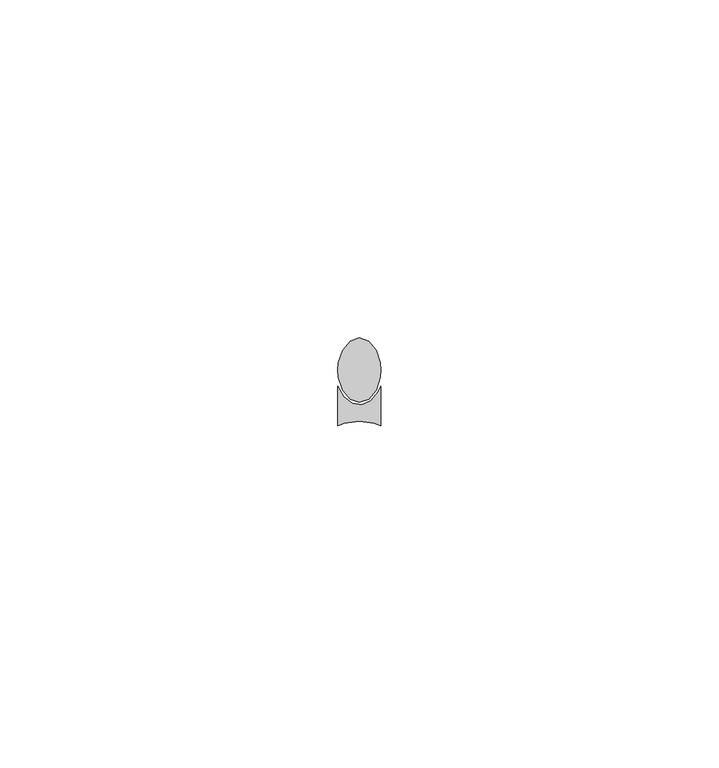
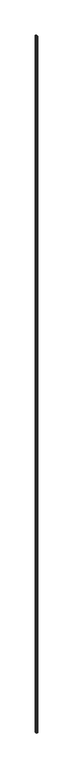
"""IFC4 building model written with IfcOpenShell, lengths in millimetres: proxy geometry, Generic Models 11:Generic Models 1:306267:Generic Models 1:306267 : Generic Models 11:Generic Models 1:306267:300405:Generic Models 1:306267:Generic Models 1:306267 : Generic Models 11:Generic Models 1:306267:300405 : Generic Models 11:Generic Models 1:306267:Generic Models 1:306267 : Generic Models 11:Generic Models 1:306267:300405:23 : Generic Models 11:Generic Models 1:306267:Generic Models 1:306267 : Generic Models 11:Generic Models 1:306267:300405:Generic Models 1:306267:Generic Models 1:306267 : Generic Models 11:Generic Models 1:306267:300405 : Generic Models 11:Generic Models 1:306267:Generic Models 1:306267 : Generic Models 11:Generic Models 1:306267:300405:300182."""

from ifc_helpers import new_model, si_unit, frame, origin, place, context, project, spatial, polyline, outline, extrude, source, transform, mapped, element, save


def generic_models_3989d67e(model_context):
    return source(origin(), model_context, "Body", "SweptSolid", [
        extrude(outline(polyline([(594928.7897638, -579082.4586403), (594927.4121829, -579082.9302761), (594926.034602, -579082.4586403), (594924.929868, -579081.1371463), (594924.3167868, -579079.2275321), (594924.2371829, -579078.1677761), (594924.3167868, -579077.1080202), (594924.929868, -579075.1984059), (594926.034602, -579073.8769119), (594927.4121829, -579073.4052761), (594928.7897638, -579073.8769119), (594929.8944979, -579075.1984059), (594930.507579, -579077.1080202), (594930.5871829, -579078.1677761), (594930.507579, -579079.2275321), (594929.8944979, -579081.1371463), (594928.7897638, -579082.4586403)])), frame((0.0, 0.0, 31.75), z_axis=(0.0, 0.0, 1.0), x_axis=(1.0, 0.0, 0.0)), (0.0, 0.0, 1.0), 3663.95),
        extrude(outline(polyline([(594925.2029461, -579086.0220872), (594924.2371829, -579086.3994958), (594924.2371829, -579080.5314037), (594925.1199717, -579082.1246204), (594926.3613558, -579083.0988254), (594927.7671321, -579083.3016133), (594929.1173799, -579082.7012598), (594930.2008653, -579081.3916847), (594930.5871829, -579080.5314037), (594930.5871829, -579086.3994958), (594929.6214197, -579086.0220872), (594927.4121829, -579085.7084011), (594925.2029461, -579086.0220872)])), frame((0.0, 0.0, 31.75), z_axis=(0.0, 0.0, 1.0), x_axis=(1.0, 0.0, 0.0)), (0.0, 0.0, 1.0), 3663.95),
    ])


if __name__ == "__main__":
    model = new_model("IFC4")
    model_context = context("Model", 3, world=origin())
    ifc_project = project(units=[si_unit("LENGTHUNIT", "METRE", prefix="MILLI")], contexts=[model_context])
    site = spatial("IfcSite", under=ifc_project)
    building = spatial("IfcBuilding", under=site)
    placement = place(None, origin())
    generic_models_shape = generic_models_3989d67e(model_context)
    element("IfcBuildingElementProxy", 1, Name="Generic Models 11:Generic Models 1:306267:Generic Models 1:306267 : Generic Models 11:Generic Models 1:306267:300405:Generic Models 1:306267:Generic Models 1:306267 : Generic Models 11:Generic Models 1:306267:300405 : Generic Models 11:Generic Models 1:306267:Generic Models 1:306267 : Generic Models 11:Generic Models 1:306267:300405:23 : Generic Models 11:Generic Models 1:306267:Generic Models 1:306267 : Generic Models 11:Generic Models 1:306267:300405:Generic Models 1:306267:Generic Models 1:306267 : Generic Models 11:Generic Models 1:306267:300405 : Generic Models 11:Generic Models 1:306267:Generic Models 1:306267 : Generic Models 11:Generic Models 1:306267:300405:300182", ObjectType="Generic Models 11:Generic Models 1:306267:Generic Models 1:306267 : Generic Models 11:Generic Models 1:306267:300405:Generic Models 1:306267:Generic Models 1:306267 : Generic Models 11:Generic Models 1:306267:300405 : Generic Models 11:Generic Models 1:306267:Generic Models 1:306267 : Generic Models 11:Generic Models 1:306267:300405:23 : Generic Models 11:Generic Models 1:306267:Generic Models 1:306267 : Generic Models 11:Generic Models 1:306267:300405:Generic Models 1:306267:Generic Models 1:306267 : Generic Models 11:Generic Models 1:306267:300405 : Generic Models 11:Generic Models 1:306267:Generic Models 1:306267 : Generic Models 11:Generic Models 1:306267:300405:300182", at=placement, inside=building, context=model_context, shape_type="MappedRepresentation", body=[
        mapped(generic_models_shape, transform((0.0, 0.0, 0.0), x_axis=(1.0, 0.0, 0.0), y_axis=(0.0, 1.0, 0.0), z_axis=(0.0, 0.0, 1.0))),
    ])
    save(model, "model.ifc")

# Revit data of these elements
# Type "Generic Models 11:Generic Models 1:306267:Generic Models 1:306267 : Generic Models 11:Generic Models 1:306267:300405:Generic Models 1:306267:Generic Models 1:306267 : Generic Models 11:Generic Models 1:306267:300405 : Generic Models 11:Generic Models 1:306267:Generic Models 1:306267 : Generic Models 11:Generic Models 1:306267:300405:23 : Generic Models 11:Generic Models 1:306267:Generic Models 1:306267 : Generic Models 11:Generic Models 1:306267:300405:Generic Models 1:306267:Generic Models 1:306267 : Generic Models 11:Generic Models 1:306267:300405 : Generic Models 11:Generic Models 1:306267:Generic Models 1:306267 : Generic Models 11:Generic Models 1:306267:300405:300182"
#   NameOverride = "Generic Models 11:Generic Models 1:306267:Generic Models 1:306267 : Generic Models 11:Generic Models 1:306267:300405:Generic Models 1:306267:Generic Models 1:306267 : Generic Models 11:Generic Models 1:306267:300405 : Generic Models 11:Generic Models 1:306267:Generic Models 1:306267 : Generic Models 11:Generic Models 1:306267:300405:300182"
#   ObjectTypeOverride = "Generic Models 1:306267:Generic Models 1:306267 : Generic Models 11:Generic Models 1:306267:300405 : Generic Models 11:Generic Models 1:306267:Generic Models 1:306267 : Generic Models 11:Generic Models 1:306267:300405"
#   Reference = "Generic Models 1"
#   Tag = "300182"
# Element 1 (IfcBuildingElementProxy, "Generic Models 11:Generic Models 1:306267:Generic Models 1:306267 : Generic Models 11:Generic Models 1:306267:300405:Generic Models 1:306267:Generic Models 1:306267 : Generic Models 11:Generic Models 1:306267:300405 : Generic Models 11:Generic Models 1:306267:Generic Models 1:306267 : Generic Models 11:Generic Models 1:306267:300405:23 : Generic Models 11:Generic Models 1:306267:Generic Models 1:306267 : Generic Models 11:Generic Models 1:306267:300405:Generic Models 1:306267:Generic Models 1:306267 : Generic Models 11:Generic Models 1:306267:300405 : Generic Models 11:Generic Models 1:306267:Generic Models 1:306267 : Generic Models 11:Generic Models 1:306267:300405:300182")
#   Materials on its faces: "SEALANT & BACKER ROD, IF NECESSARY"
# Materials
#   "SEALANT & BACKER ROD, IF NECESSARY": class "Unassigned", colour RGB 120 120 120, transparency 0, Cost = 0
